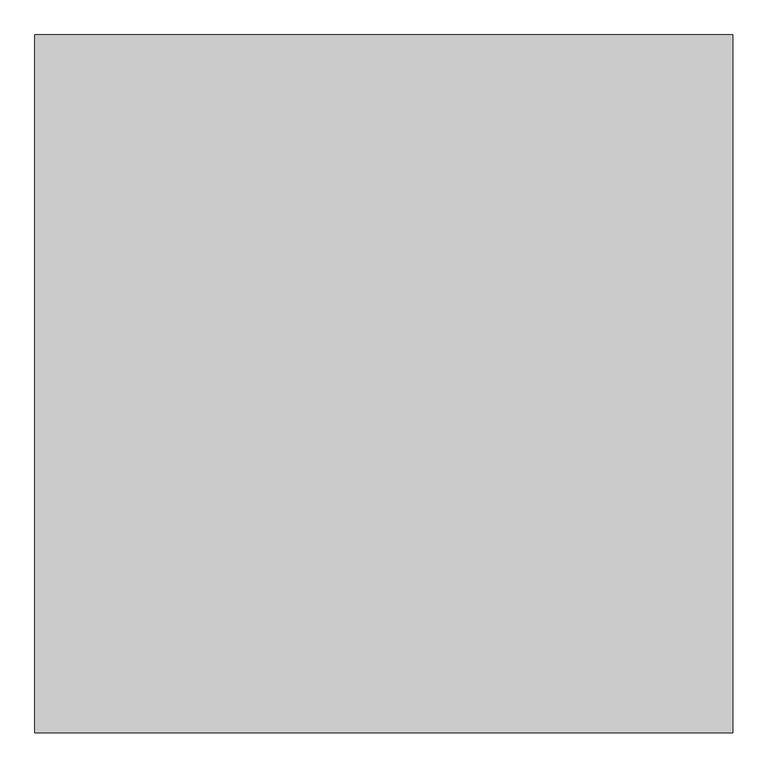
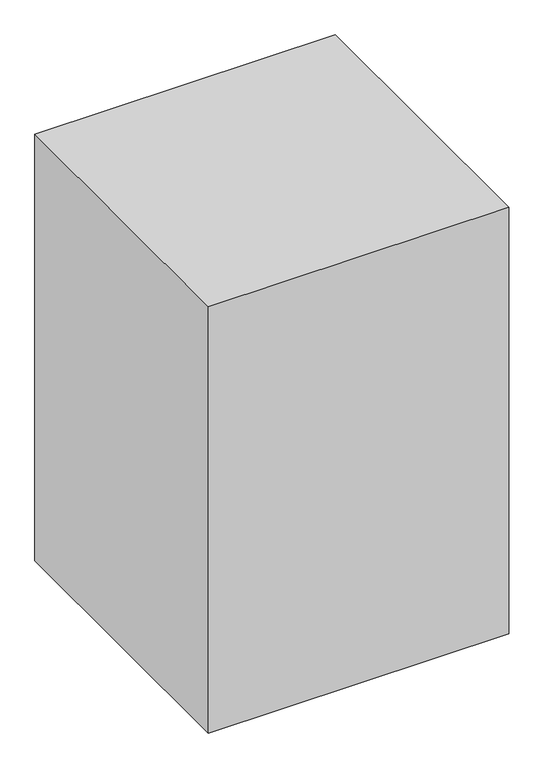
"""IFC4 building model written with IfcOpenShell, lengths in millimetres: proxy geometry, Space Planning Box_hec : Space Planning Box_hec."""

import ifcopenshell
import ifcopenshell.guid

model = None  # the IFC model being written
_history = None  # IfcOwnerHistory: only IFC2X3 demands one
_inside = {}  # id of a spatial element -> (the spatial element, [elements in it])
_under = {}  # id of a project, library or spatial element -> (it, [spatial elements below it])
_declared = {}  # id of a project -> (the project, [libraries it declares])
_typed = {}  # id of a type object -> (the type object, [elements of that type])
_made_of = {}  # id of a material, layer set ... -> (it, [elements and type objects made of it])


def new_model(schema):
    """Start an empty IFC model of exactly this schema.

    Asked for "IFC4X3", IfcOpenShell would pick the latest addendum, in which some entities
    have other attributes; the version numbers below select the first issue.
    IFC2X3 requires an IfcOwnerHistory on every rooted entity: one is made here for all.
    """
    global model, _history
    if schema == "IFC4X3":
        model = ifcopenshell.file(schema_version=(4, 3, 0, 0))
    else:
        model = ifcopenshell.file(schema=schema)
    _inside.clear()
    _under.clear()
    _declared.clear()
    _typed.clear()
    _made_of.clear()
    _history = None
    if model.schema == "IFC2X3":
        org = make("IfcOrganization", Name="unknown")
        user = make(
            "IfcPersonAndOrganization",
            ThePerson=make("IfcPerson", FamilyName="unknown"),
            TheOrganization=org,
        )
        app = make(
            "IfcApplication",
            ApplicationDeveloper=org,
            Version="unknown",
            ApplicationFullName="unknown",
            ApplicationIdentifier="unknown",
        )
        _history = make(
            "IfcOwnerHistory",
            OwningUser=user,
            OwningApplication=app,
            ChangeAction="ADDED",
            CreationDate=0,
        )
    return model


def make(cls, **values):
    """One entity of the class cls with the attributes given. An attribute that is None is left unset."""
    return model.create_entity(
        cls, **{name: value for name, value in values.items() if value is not None}
    )


def rooted(cls, **values):
    """An entity with a GlobalId (a new one), such as an element, a storey or a relation."""
    return make(cls, GlobalId=ifcopenshell.guid.new(), OwnerHistory=_history, **values)


def si_unit(unit_type, name, prefix=None):
    """IfcSIUnit, for example si_unit("LENGTHUNIT", "METRE", prefix="MILLI")."""
    return make("IfcSIUnit", UnitType=unit_type, Prefix=prefix, Name=name)


def assignment(units):
    """IfcUnitAssignment: the units of a project."""
    return None if units is None else make("IfcUnitAssignment", Units=units)


def point(xyz):
    """IfcCartesianPoint."""
    return None if xyz is None else make("IfcCartesianPoint", Coordinates=xyz)


def direction(xyz):
    """IfcDirection."""
    return None if xyz is None else make("IfcDirection", DirectionRatios=xyz)


def frame(location, z_axis=None, x_axis=None):
    """IfcAxis2Placement3D, a coordinate frame: its origin and axes. An axis left out is left unset."""
    return make(
        "IfcAxis2Placement3D",
        Location=point(location),
        Axis=direction(z_axis),
        RefDirection=direction(x_axis),
    )


def origin():
    """The frame at (0, 0, 0) with its axes left unset."""
    return frame((0.0, 0.0, 0.0))


def origin_with_axes():
    """The frame at (0, 0, 0) with the z axis (0, 0, 1) and the x axis (1, 0, 0) written out."""
    return frame((0.0, 0.0, 0.0), z_axis=(0.0, 0.0, 1.0), x_axis=(1.0, 0.0, 0.0))


def place(relative_to, where):
    """IfcLocalPlacement: puts the frame where relative to a parent placement (None: the world)."""
    return make(
        "IfcLocalPlacement", PlacementRelTo=relative_to, RelativePlacement=where
    )


def context(
    kind, dimensions, precision=None, world=None, true_north=None, identifier=None
):
    """IfcGeometricRepresentationContext, for example the 3D "Model" context."""
    return make(
        "IfcGeometricRepresentationContext",
        ContextIdentifier=identifier,
        ContextType=kind,
        CoordinateSpaceDimension=dimensions,
        Precision=precision,
        WorldCoordinateSystem=world,
        TrueNorth=true_north,
    )


def project(units=None, contexts=None):
    """IfcProject with its units and contexts."""
    return rooted(
        "IfcProject",
        Name="project",
        RepresentationContexts=contexts,
        UnitsInContext=assignment(units),
    )


def spatial(cls, under=None, at=None, **own):
    """A site, building, storey or space (cls), placed at a placement, below another one or the project."""
    s = rooted(cls, ObjectPlacement=at, **own)
    if under is not None:
        _under.setdefault(under.id(), (under, []))[1].append(s)
    return s


def polyline(points):
    """IfcPolyline through the points."""
    return make("IfcPolyline", Points=[point(p) for p in points])


def outline(outer, holes=None, kind="AREA"):
    """IfcArbitraryClosedProfileDef: a profile drawn as a closed curve; with holes, ...WithVoids."""
    if holes is None:
        return make("IfcArbitraryClosedProfileDef", ProfileType=kind, OuterCurve=outer)
    return make(
        "IfcArbitraryProfileDefWithVoids",
        ProfileType=kind,
        OuterCurve=outer,
        InnerCurves=holes,
    )


def extrude(swept, where, along, depth):
    """IfcExtrudedAreaSolid: the profile swept, set in the frame where, extruded along a direction by depth."""
    return make(
        "IfcExtrudedAreaSolid",
        SweptArea=swept,
        Position=where,
        ExtrudedDirection=direction(along),
        Depth=depth,
    )


def shape(context_of_items, identifier, shape_type, items):
    """IfcShapeRepresentation: the items that make up one representation, for example the "Body"."""
    return make(
        "IfcShapeRepresentation",
        ContextOfItems=context_of_items,
        RepresentationIdentifier=identifier,
        RepresentationType=shape_type,
        Items=items,
    )


def source(mapping_origin, context_of_items, identifier, shape_type, items):
    """IfcRepresentationMap: a shape defined once, which mapped items show again and again."""
    return make(
        "IfcRepresentationMap",
        MappingOrigin=mapping_origin,
        MappedRepresentation=shape(context_of_items, identifier, shape_type, items),
    )


def transform(
    local_origin,
    x_axis=None,
    y_axis=None,
    z_axis=None,
    scale=None,
    scale2=None,
    scale3=None,
    uniform=True,
):
    """IfcCartesianTransformationOperator3D, or its non-uniform kind. x_axis, y_axis, z_axis: its Axis1, 2, 3."""
    if uniform:
        return make(
            "IfcCartesianTransformationOperator3D",
            Axis1=direction(x_axis),
            Axis2=direction(y_axis),
            LocalOrigin=point(local_origin),
            Scale=scale,
            Axis3=direction(z_axis),
        )
    return make(
        "IfcCartesianTransformationOperator3DnonUniform",
        Axis1=direction(x_axis),
        Axis2=direction(y_axis),
        LocalOrigin=point(local_origin),
        Scale=scale,
        Axis3=direction(z_axis),
        Scale2=scale2,
        Scale3=scale3,
    )


def mapped(mapping_source, mapping_target):
    """IfcMappedItem: shows the shape of a source again, moved by a transform."""
    return make(
        "IfcMappedItem", MappingSource=mapping_source, MappingTarget=mapping_target
    )


def made_of(thing, what):
    """Note that an element or type object is made of a material, layer set ...; save() writes the relation."""
    if what is not None:
        _made_of.setdefault(what.id(), (what, []))[1].append(thing)
    return thing


def element(
    cls,
    number,
    at=None,
    inside=None,
    cuts=None,
    type_object=None,
    material=None,
    context=None,
    identifier="Body",
    shape_type=None,
    held_by="IfcProductDefinitionShape",
    body=None,
    shapes=None,
    **own,
):
    """One element of the class cls, such as IfcWall. Its Tag is "e" and its number.

    at: its placement. inside: the storey or other place that contains it. cuts: it is an
    opening in that element (IfcRelVoidsElement). A single representation is given by context,
    identifier, shape_type and body (its items); several are given by shapes. held_by: the class
    of the entity that holds the representations. save() writes the other relations.
    """
    e = rooted(cls, Tag="e%d" % number, ObjectPlacement=at, **own)
    if body is not None:
        shapes = [shape(context, identifier, shape_type, body)]
    if shapes is not None:
        e.Representation = make(held_by, Representations=shapes)
    if inside is not None:
        _inside.setdefault(inside.id(), (inside, []))[1].append(e)
    if cuts is not None:
        rooted(
            "IfcRelVoidsElement", RelatingBuildingElement=cuts, RelatedOpeningElement=e
        )
    if type_object is not None:
        _typed.setdefault(type_object.id(), (type_object, []))[1].append(e)
    return made_of(e, material)


def aggregate(whole, parts):
    """IfcRelAggregates: a whole, such as a stair, and the parts it consists of."""
    return rooted("IfcRelAggregates", RelatingObject=whole, RelatedObjects=parts)


def save(model, path):
    """Write the relations noted so far, then the file.

    IfcRelAggregates (storeys below a building ...), IfcRelContainedInSpatialStructure (elements
    in a storey), IfcRelDefinesByType, IfcRelAssociatesMaterial and IfcRelDeclares: one each for
    every whole, place, type object, material and project.
    """
    for whole, parts in _under.values():
        aggregate(whole, parts)
    for where, things in _inside.values():
        rooted(
            "IfcRelContainedInSpatialStructure",
            RelatedElements=things,
            RelatingStructure=where,
        )
    for kind, things in _typed.values():
        rooted("IfcRelDefinesByType", RelatedObjects=things, RelatingType=kind)
    for what, things in _made_of.values():
        rooted("IfcRelAssociatesMaterial", RelatedObjects=things, RelatingMaterial=what)
    for by, libraries in _declared.values():
        rooted("IfcRelDeclares", RelatingContext=by, RelatedDefinitions=libraries)
    model.write(path)


def generic_models_7bff30ad(model_context):
    return source(origin(), model_context, "Body", "SweptSolid", [
        extrude(outline(polyline([(2000.0, 2000.0), (2000.0, -2000.0), (-2000.0, -2000.0), (-2000.0, 2000.0), (2000.0, 2000.0)])), origin_with_axes(), (0.0, 0.0, 1.0), 6000.0),
    ])


if __name__ == "__main__":
    model = new_model("IFC4")
    model_context = context("Model", 3, world=origin())
    ifc_project = project(units=[si_unit("LENGTHUNIT", "METRE", prefix="MILLI")], contexts=[model_context])
    site = spatial("IfcSite", under=ifc_project)
    building = spatial("IfcBuilding", under=site)
    placement = place(None, origin())
    generic_models_shape = generic_models_7bff30ad(model_context)
    element("IfcBuildingElementProxy", 1, Name="Space Planning Box_hec : Space Planning Box_hec", ObjectType="Space Planning Box_hec : Space Planning Box_hec", at=placement, inside=building, context=model_context, shape_type="MappedRepresentation", body=[
        mapped(generic_models_shape, transform((0.0, 0.0, 0.0), x_axis=(1.0, 0.0, 0.0), y_axis=(0.0, 1.0, 0.0), z_axis=(0.0, 0.0, 1.0))),
    ])
    save(model, "model.ifc")

# Revit data of these elements
# Project information
#   Project Issue Date = "Issue Date"
#   Project Status = "Project Status"
#   Client Name = "Owner"
#   Project Address = "Enter address here"
#   Project Name = "Project Name"
#   Project Number = "Project Number"
# Type "Space Planning Box_hec : Space Planning Box_hec"
#   Type Comments = "..."
#   Room Name [instance default] = "?"
#   Interior Finish [instance default] = ""
#   Exterior Finish [instance default] = ""
#   Department [instance default] = ""
#   Assembly Code = "..."
#   Width [instance default] = 1524 mm
#   Program Area [instance default] = 0 m²
#   Length [instance default] = 1524 mm
#   Height [instance default] = 1524 mm
#   Area [instance default] = 2.32258 m²
#   Fill Color [instance default] = Cyan
#   Default Elevation = 0
# Element 1 (IfcBuildingElementProxy, "Space Planning Box_hec : Space Planning Box_hec")
#   Room Name = "Toilet (F)"
#   Interior Finish = "IF5"
#   Exterior Finish = "EF1"
#   Department = "AR"
#   Width = 4000 mm
#   Program Area = 72 m²
#   Length = 4000 mm
#   Height = 6000 mm
#   Area = 16 m²
#   Fill Color = Lavender
#   Materials on its faces: "Lavender"
# Materials
#   "Cyan": class "Generic", colour RGB 0 255 255, transparency 0.2, Cost = 0
#   "Lavender": class "Generic", colour RGB 186 85 211, transparency 0.2, Cost = 0
